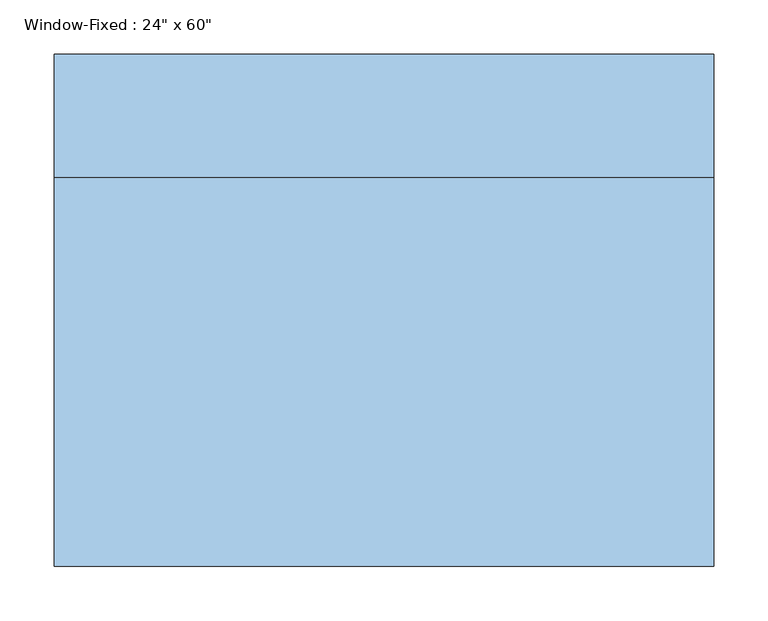
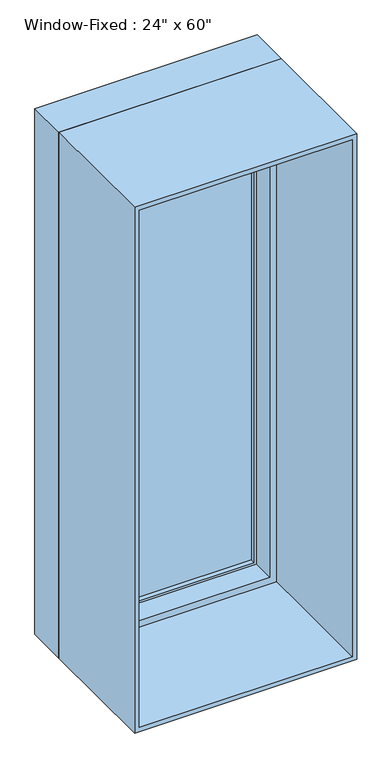
"""IFC4 building model written with IfcOpenShell, lengths in millimetres: window geometry."""

from ifc_helpers import new_model, si_unit, frame, origin, place, context, project, spatial, polyline, outline, extrude, faceted_brep, source, transform, mapped, element, save


def window_69ce9bab(model_context):
    return source(origin(), model_context, "Body", "SolidModel", [
        extrude(outline(polyline([(266.7, 227.0125), (266.7, 220.6625), (-266.7, 220.6625), (-266.7, 227.0125), (266.7, 227.0125)])), frame((0.0, 0.0, 952.5), z_axis=(0.0, 0.0, 1.0), x_axis=(1.0, 0.0, 0.0)), (0.0, 0.0, 1.0), 1447.8),
        extrude(outline(polyline([(-266.7, 207.9625), (-266.7, 214.3125), (266.7, 214.3125), (266.7, 207.9625), (-266.7, 207.9625)])), frame((0.0, 0.0, 952.5), z_axis=(0.0, 0.0, 1.0), x_axis=(1.0, 0.0, 0.0)), (0.0, 0.0, 1.0), 1447.8),
        extrude(outline(polyline([(927.1, 292.1), (2425.7, 292.1), (2425.7, -292.1), (927.1, -292.1), (927.1, 292.1)]), holes=[polyline([(952.5, -266.7), (2400.3, -266.7), (2400.3, 266.7), (952.5, 266.7), (952.5, -266.7)])]), frame((0.0, 195.2625, 0.0), z_axis=(0.0, 1.0, 0.0), x_axis=(0.0, 0.0, 1.0)), (0.0, 0.0, 1.0), 44.45),
        extrude(outline(polyline([(2438.4, -304.8), (914.4, -304.8), (914.4, 304.8), (2438.4, 304.8), (2438.4, -304.8)]), holes=[polyline([(2425.7, 292.1), (927.1, 292.1), (927.1, -292.1), (2425.7, -292.1), (2425.7, 292.1)])]), frame((0.0, -227.0125, 0.0), z_axis=(0.0, 1.0, 0.0), x_axis=(0.0, 0.0, 1.0)), (0.0, 0.0, 1.0), 358.775),
        faceted_brep([(304.8, 131.7625, 2438.4), (304.8, 246.0625, 2438.4), (-304.8, 246.0625, 2438.4), (-304.8, 131.7625, 2438.4), (-304.8, 246.0625, 914.4), (-304.8, 131.7625, 914.4), (304.8, 246.0625, 914.4), (304.8, 131.7625, 914.4), (273.05, 131.7625, 2406.65), (273.05, 131.7625, 946.15), (-273.05, 131.7625, 946.15), (-273.05, 131.7625, 2406.65), (-292.1, 246.0625, 2425.7), (-292.1, 246.0625, 927.1), (292.1, 246.0625, 927.1), (292.1, 246.0625, 2425.7), (273.05, 195.2625, 2406.65), (-273.05, 195.2625, 2406.65), (292.1, 195.2625, 2425.7), (-292.1, 195.2625, 2425.7), (-273.05, 195.2625, 946.15), (-292.1, 195.2625, 927.1), (273.05, 195.2625, 946.15), (292.1, 195.2625, 927.1)], [[[0, 1, 2, 3]], [[3, 2, 4, 5]], [[5, 4, 6, 7]], [[3, 5, 7, 0], [8, 9, 10, 11]], [[7, 6, 1, 0]], [[1, 6, 4, 2], [12, 13, 14, 15]], [[16, 8, 11, 17]], [[15, 18, 19, 12]], [[17, 11, 10, 20]], [[12, 19, 21, 13]], [[20, 10, 9, 22]], [[13, 21, 23, 14]], [[22, 9, 8, 16]], [[18, 23, 21, 19], [17, 20, 22, 16]], [[14, 23, 18, 15]]]),
    ])


if __name__ == "__main__":
    model = new_model("IFC4")
    model_context = context("Model", 3, world=origin())
    ifc_project = project(units=[si_unit("LENGTHUNIT", "METRE", prefix="MILLI")], contexts=[model_context])
    site = spatial("IfcSite", under=ifc_project)
    building = spatial("IfcBuilding", under=site)
    placement = place(None, origin())
    window_shape = window_69ce9bab(model_context)
    element("IfcWindow", 1, ObjectType="Window-Fixed : 24\" x 60\"", at=placement, inside=building, context=model_context, shape_type="MappedRepresentation", body=[
        mapped(window_shape, transform((0.0, 0.0, 0.0), x_axis=(1.0, 0.0, 0.0), y_axis=(0.0, 1.0, 0.0), z_axis=(0.0, 0.0, 1.0))),
    ])
    save(model, "model.ifc")

# Revit data of these elements
# Type "Window-Fixed : 24\" x 60\""
#   Type Mark = "WT-21"
#   Fire Rating = "0.5h"
#   Assembly Code = "B2020100"
#   Analytic Construction = "Double glazing - domestic"
#   Window Inset [instance default] = 0' - 0"
#   Wall Thickness [instance default] = 0' - 6"
#   Visual Light Transmittance = 0.81
#   Thermal Resistance (R) = 1.8146 (h·ft²·°F)/BTU
#   Solar Heat Gain Coefficient = 0.76
#   Rough Width = 2' - 0 1/2"
#   Rough Height = 5' - 0 1/2"
#   Interior Wall Closure [instance default] = 0' - 2 1/4"
#   Height = 5' - 0"
#   Heat Transfer Coefficient (U) = 0.5511 BTU/(h·ft²·°F)
#   Frame Extension [instance default] = 0' - 0 1/4"
#   Exterior Wall Closure [instance default] = 0' - 1 1/4"
#   Extension Jamb [instance default] = 0' - 2 1/4"
#   Default Sill Height = 3' - 0"
#   Width = 2' - 0"
#   Muntin Visibility = no
#   Interior Trim Visibility [instance default] = yes
#   Exterior Trim Visibility [instance default] = yes
#   Extension Jamb Visibility [instance default] = yes
#   Muntin Pattern = Muntin Pattern_2x2 : Muntin Pattern_2x2
#   Interior Trim Material = Wood - Stained
#   Interior Trim = Trim-Window-Interior-Flat : Picture Frame
#   Interior Frame Material = Wood - Stained
#   Glass Panel Material = Glass
#   Exterior Trim Material = Clad - White
#   Exterior Trim = Trim-Window-Exterior-Flat : with Sill
#   Exterior Frame Material = Clad - White
#   Wall Closure = (empty or 0)
# Element 1 (IfcWindow, "Window-Fixed : 24\" x 60\"")
#   Wall Thickness = 1' - 5 7/8"
#   Extension Jamb = 1' - 2 1/8"
#   Materials on its faces: "Wood - Stained", "Glass", "Clad - White"
# Materials
#   "Wood - Stained": class "Wood", colour RGB 224 178 126, transparency 0, Cost = 0
#   "Glass": class "Glass", colour RGB 0 128 192, transparency 0.75, Description = "Soda Lime Glass", Cost = 0
#   "Clad - White": class "Wood", colour RGB 242 242 238, transparency 0, Cost = 0
